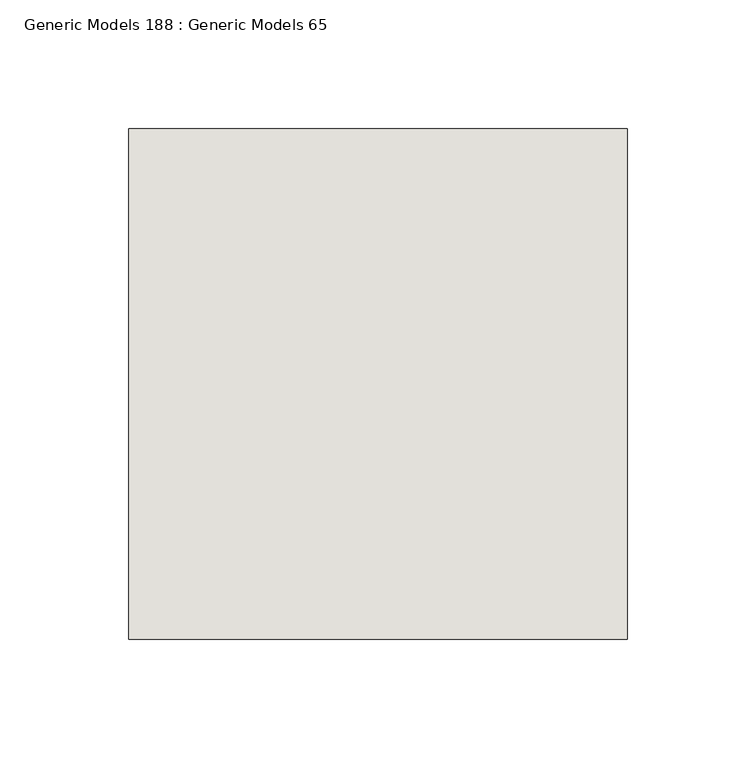
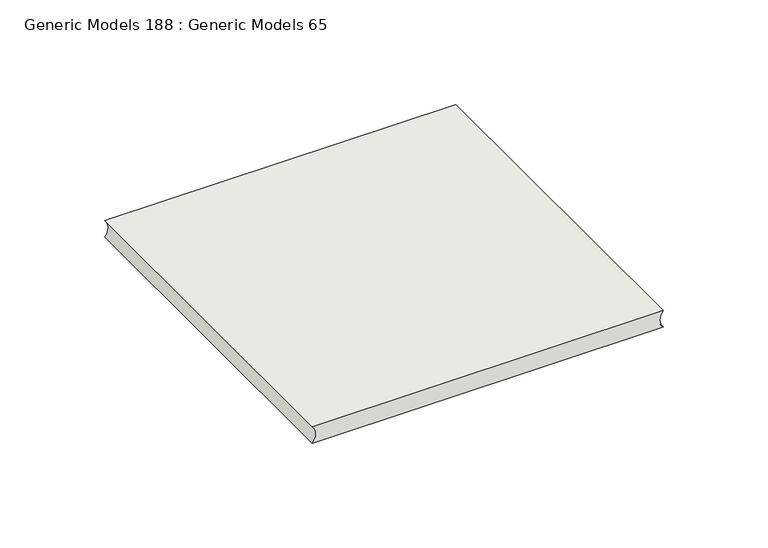
"""IFC4 building model written with IfcOpenShell, lengths in millimetres: wall geometry, Generic Models 188 : Generic Models 65."""

from ifc_helpers import new_model, si_unit, point, frame, frame_2d, origin, place, context, project, spatial, polyline, circle_curve, trimmed, segment, composite_curve, outline, extrude, source, transform, mapped, element, save


def generic_models_188_generic_models_65_5e3e2d01(model_context):
    return source(origin(), model_context, "Body", "SweptSolid", [
        extrude(outline(composite_curve([segment(polyline([(2193.3712588, 375199.1901825), (2193.3712588, 375005.5151825)]), True, "CONTINUOUS"), segment(trimmed(circle_curve(frame_2d((2188.6087588, 375000.6321853)), 6.8209287), [point((2193.3712588, 375005.5151825))], [point((2183.8462588, 375005.5151825))], True, "CARTESIAN"), True, "CONTINUOUS"), segment(polyline([(2183.8462588, 375005.5151825), (2183.8462588, 375199.1901825)]), True, "CONTINUOUS"), segment(trimmed(circle_curve(frame_2d((2188.6087588, 375204.0731798)), 6.8209287), [point((2183.8462588, 375199.1901825))], [point((2193.3712588, 375199.1901825))], True, "CARTESIAN"), True, "CONTINUOUS")], self_intersect=False)), frame((0.0, 490.5375, 0.0), z_axis=(0.0, 1.0, 0.0), x_axis=(0.0, 0.0, 1.0)), (0.0, 0.0, 1.0), 198.4375),
    ])


if __name__ == "__main__":
    model = new_model("IFC4")
    model_context = context("Model", 3, world=origin())
    ifc_project = project(units=[si_unit("LENGTHUNIT", "METRE", prefix="MILLI")], contexts=[model_context])
    site = spatial("IfcSite", under=ifc_project)
    building = spatial("IfcBuilding", under=site)
    placement = place(None, origin())
    generic_models_188_generic_models_65_shape = generic_models_188_generic_models_65_5e3e2d01(model_context)
    element("IfcWall", 1, ObjectType="Generic Models 188 : Generic Models 65", at=placement, inside=building, context=model_context, shape_type="MappedRepresentation", body=[
        mapped(generic_models_188_generic_models_65_shape, transform((0.0, 0.0, 0.0), x_axis=(1.0, 0.0, 0.0), y_axis=(0.0, 1.0, 0.0), z_axis=(0.0, 0.0, 1.0))),
    ])
    save(model, "model.ifc")

# Revit data of these elements
# Element 1 (IfcWall, "Generic Models 188 : Generic Models 65")
#   Materials on its faces: "MORTAR JOINT"
# Materials
#   "MORTAR JOINT": class "Generic", colour RGB 120 120 120, transparency 0, Cost = 0
